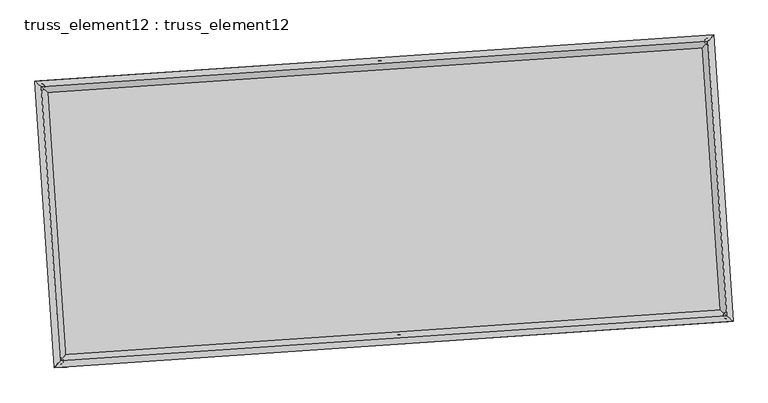
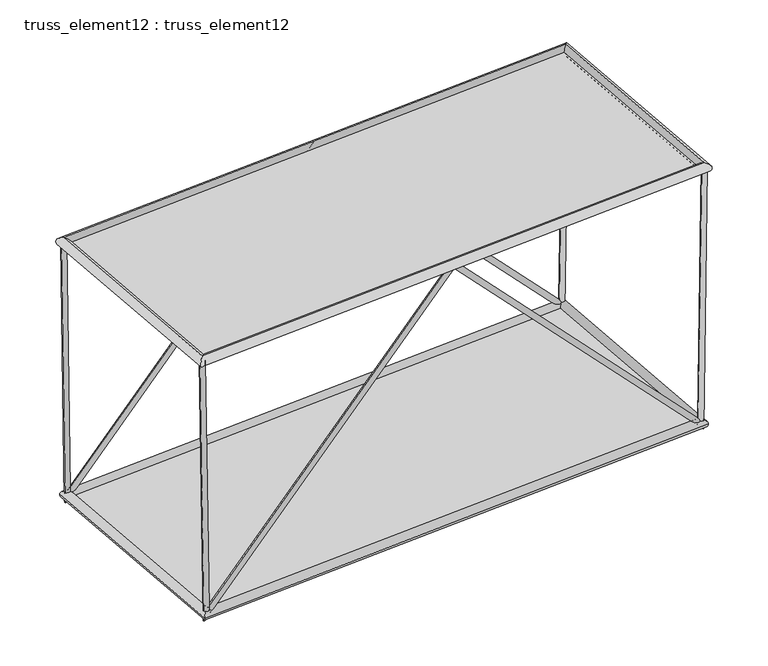
"""IFC4 building model written with IfcOpenShell, lengths in millimetres: plate geometry, truss_element12 : truss_element12."""

from ifc_helpers import new_model, si_unit, frame, origin, origin_with_axes, place, context, project, spatial, polyline, circle_curve, ellipse_curve, outline, extrude, source, transform, mapped, element, save
from ifc_brep_helpers import plane_surface, cylinder_surface, advanced_brep


def truss_element12_truss_element12_87516094(model_context):
    return source(origin(), model_context, "Body", "SolidModel", [
        advanced_brep(
        [(-3739.4843414, 2271.1412017, 5000.1872867), (-3838.5765897, 2257.7806857, 4998.6963313), (-3666.7596998, 2276.1000186, 122.3078972), (-3762.227183, 2262.9866615, -122.3078972), (1063.0583794, 2598.6083337, 5071.5713796), (1063.5164535, 2592.0357757, 4927.3317201), (5794.1667617, 2921.2046296, 122.3170383), (5890.5942153, 2921.1758589, -122.3170383), (5865.6107768, 2926.0761254, 5000.1936444), (5965.5998202, 2926.2902059, 4998.7289371)],
        [
            (0, 1, circle_curve(frame((-3789.0304655, 2264.4609437, 4999.441809), z_axis=(-0.01490740482663817, -0.0010164792667785262, 0.999888361794073), x_axis=(-0.13360539978853184, 0.9910341205011933, -0.0009844540481966856)), 50.0)),
            (1, 0, circle_curve(frame((-3789.0304655, 2264.4609437, 4999.441809), z_axis=(-0.01490740482663817, -0.0010164792667785262, 0.999888361794073), x_axis=(-0.13360539978853184, 0.9910341205011933, -0.0009844540481966856)), 50.0)),
            (0, 2),
            (2, 3, ellipse_curve(frame((-3714.4934414, 2269.54334, 0.0), z_axis=(-0.9285444803963763, -0.06331391839020976, 0.3657820329971138), x_axis=(0.3649346609037332, 0.024883507280505895, 0.93070054493188)), 131.701033, 50.0)),
            (3, 1),
            (3, 2, ellipse_curve(frame((-3714.4934414, 2269.54334, 0.0), z_axis=(-0.9285444803963763, -0.06331391839020976, 0.3657820329971138), x_axis=(0.3649346609037332, 0.024883507280505895, 0.93070054493188)), 131.701033, 50.0)),
            (2, 4),
            (4, 5, ellipse_curve(frame((1063.2874165, 2595.3220547, 4999.4515499), z_axis=(-0.9976833937280465, -0.06802823806868136, -6.858978492521302e-05), x_axis=(6.843088956005366e-05, 4.666042230024793e-06, -0.9999999976477206)), 72.2768712, 50.0)),
            (5, 3),
            (5, 4, ellipse_curve(frame((1063.2874165, 2595.3220547, 4999.4515499), z_axis=(-0.9976833937280465, -0.06802823806868136, -6.858978492521302e-05), x_axis=(6.843088956005366e-05, 4.666042230024793e-06, -0.9999999976477206)), 72.2768712, 50.0)),
            (4, 6),
            (6, 7, ellipse_curve(frame((5842.3804885, 2921.1902443, 0.0), z_axis=(-0.9284714273096886, -0.06330893717792861, -0.36596828707267914), x_axis=(-0.3651204835023758, -0.02489617781713149, 0.9306273222171639)), 131.7212392, 50.0)),
            (7, 5),
            (7, 6, ellipse_curve(frame((5842.3804885, 2921.1902443, 0.0), z_axis=(-0.9284714273096886, -0.06330893717792861, -0.36596828707267914), x_axis=(-0.3651204835023758, -0.02489617781713149, 0.9306273222171639)), 131.7212392, 50.0)),
            (8, 9, circle_curve(frame((5915.6052985, 2926.1831657, 4999.4612908), z_axis=(0.0146449619914404, 0.0009985842874829112, 0.9998922581546925), x_axis=(-0.0021552007044751543, 0.9999972098877479, -0.0009671228685221853)), 50.0)),
            (9, 8, circle_curve(frame((5915.6052985, 2926.1831657, 4999.4612908), z_axis=(0.0146449619914404, 0.0009985842874829112, 0.9998922581546925), x_axis=(-0.0021552007044751543, 0.9999972098877479, -0.0009671228685221853)), 50.0)),
            (6, 8),
            (9, 7),
        ],
        [
            plane_surface(frame((-3789.0304655, 2314.4609179, 4999.4926386), z_axis=(-0.014907404826640259, -0.0010164792667773047, 0.9998883617940729), x_axis=(0.9998888784666697, -1.5154751946688795e-05, 0.014907397123536715))),
            cylinder_surface(frame((-3789.0304655, 2264.4609437, 4999.441809), z_axis=(-0.01490740482663817, -0.0010164792667785262, 0.999888361794073), x_axis=(-0.13360539978853184, 0.9910341205011933, -0.0009844540481966856)), 50.0),
            cylinder_surface(frame((-3714.4934414, 2269.54334, 0.0), z_axis=(-0.6901322286195807, -0.04705749323136387, -0.7221517149126984), x_axis=(-0.020411728114871647, 0.9987523666831909, -0.04557489879406897)), 50.0),
            cylinder_surface(frame((1063.2874165, 2595.3220547, 4999.4515499), z_axis=(-0.6902310570943108, -0.04706423196937507, 0.722056816248973), x_axis=(-0.11534289058656251, 0.9922793715813788, -0.04558142522124768)), 50.0),
            plane_surface(frame((5915.6052985, 2876.1831906, 4999.5112253), z_axis=(0.014644961991439494, 0.000998584287486898, 0.9998922581546924), x_axis=(0.999892756793582, -1.462579745314941e-05, -0.014644954688108676))),
            cylinder_surface(frame((5842.3804885, 2921.1902443, 0.0), z_axis=(-0.0146449619914404, -0.0009985842874829112, -0.9998922581546925), x_axis=(-0.0021552007044751543, 0.9999972098877479, -0.0009671228685221853)), 50.0),
        ],
        [
            (0, [[1, 2]]),
            (1, [[-1, 3, 4, 5]]),
            (1, [[-2, -5, 6, -3]]),
            (2, [[-4, 7, 8, 9]]),
            (2, [[-6, -9, 10, -7]]),
            (3, [[-8, 11, 12, 13]]),
            (3, [[-10, -13, 14, -11]]),
            (4, [[15, 16]]),
            (5, [[-12, 17, -16, 18]]),
            (5, [[-14, -18, -15, -17]]),
        ],
    ),
        advanced_brep(
        [(-3467.3713885, -1719.5923826, 5000.1872867), (-3566.4636368, -1732.9528986, 4998.6963313), (-3394.6467469, -1714.6335657, 122.3078972), (-3490.1142301, -1727.7469228, -122.3078972), (1335.1713323, -1392.1252506, 5071.5713796), (1335.6294064, -1398.6978086, 4927.3317201), (6066.2797147, -1069.5289547, 122.3170383), (6162.7071682, -1069.5577254, -122.3170383), (6137.7237297, -1064.6574589, 5000.1936444), (6237.7127731, -1064.4433784, 4998.7289371)],
        [
            (0, 1, circle_curve(frame((-3516.9175126, -1726.2726406, 4999.441809), z_axis=(-0.014907404826637962, -0.0010164792667784767, 0.999888361794073), x_axis=(-0.13360539978853184, 0.9910341205011933, -0.0009844540481967064)), 50.0)),
            (1, 0, circle_curve(frame((-3516.9175126, -1726.2726406, 4999.441809), z_axis=(-0.014907404826637962, -0.0010164792667784767, 0.999888361794073), x_axis=(-0.13360539978853184, 0.9910341205011933, -0.0009844540481967064)), 50.0)),
            (0, 2),
            (2, 3, ellipse_curve(frame((-3442.3804885, -1721.1902443, 0.0), z_axis=(-0.9285444803963764, -0.0633139183902097, 0.36578203299711326), x_axis=(0.36493466090373267, 0.024883507280505864, 0.9307005449318803)), 131.701033, 50.0)),
            (3, 1),
            (3, 2, ellipse_curve(frame((-3442.3804885, -1721.1902443, 0.0), z_axis=(-0.9285444803963764, -0.0633139183902097, 0.36578203299711326), x_axis=(0.36493466090373267, 0.024883507280505864, 0.9307005449318803)), 131.701033, 50.0)),
            (2, 4),
            (4, 5, ellipse_curve(frame((1335.4003694, -1395.4115296, 4999.4515499), z_axis=(-0.9976833937280466, -0.06802823806868125, -6.858978492569457e-05), x_axis=(6.843088956082234e-05, 4.6660422299959605e-06, -0.9999999976477206)), 72.2768712, 50.0)),
            (5, 3),
            (5, 4, ellipse_curve(frame((1335.4003694, -1395.4115296, 4999.4515499), z_axis=(-0.9976833937280466, -0.06802823806868125, -6.858978492569457e-05), x_axis=(6.843088956082234e-05, 4.6660422299959605e-06, -0.9999999976477206)), 72.2768712, 50.0)),
            (4, 6),
            (6, 7, ellipse_curve(frame((6114.4934414, -1069.54334, 0.0), z_axis=(-0.9284714273096886, -0.06330893717792847, -0.36596828707267864), x_axis=(-0.3651204835023754, -0.024896177817131368, 0.930627322217164)), 131.7212392, 50.0)),
            (7, 5),
            (7, 6, ellipse_curve(frame((6114.4934414, -1069.54334, 0.0), z_axis=(-0.9284714273096886, -0.06330893717792847, -0.36596828707267864), x_axis=(-0.3651204835023754, -0.024896177817131368, 0.930627322217164)), 131.7212392, 50.0)),
            (8, 9, circle_curve(frame((6187.7182514, -1064.5504186, 4999.4612908), z_axis=(0.014644961991440565, 0.0009985842874829474, 0.9998922581546924), x_axis=(-0.0021552007044752385, 0.999997209887748, -0.0009671228685222203)), 50.0)),
            (9, 8, circle_curve(frame((6187.7182514, -1064.5504186, 4999.4612908), z_axis=(0.014644961991440565, 0.0009985842874829474, 0.9998922581546924), x_axis=(-0.0021552007044752385, 0.999997209887748, -0.0009671228685222203)), 50.0)),
            (6, 8),
            (9, 7),
        ],
        [
            plane_surface(frame((-3516.9175126, -1676.2726664, 4999.4926386), z_axis=(-0.014907404826640259, -0.001016479266777302, 0.9998883617940729), x_axis=(0.9998888784666697, -1.5154751946688795e-05, 0.014907397123536715))),
            cylinder_surface(frame((-3516.9175126, -1726.2726406, 4999.441809), z_axis=(-0.014907404826637962, -0.0010164792667784767, 0.999888361794073), x_axis=(-0.13360539978853184, 0.9910341205011933, -0.0009844540481967064)), 50.0),
            cylinder_surface(frame((-3442.3804885, -1721.1902443, 0.0), z_axis=(-0.6901322286195796, -0.04705749323136377, -0.7221517149126994), x_axis=(-0.020411728114871578, 0.9987523666831909, -0.04557489879406886)), 50.0),
            cylinder_surface(frame((1335.4003694, -1395.4115296, 4999.4515499), z_axis=(-0.6902310570943105, -0.047064231969374926, 0.7220568162489734), x_axis=(-0.11534289058656241, 0.9922793715813789, -0.04558142522124771)), 50.0),
            plane_surface(frame((6187.7182514, -1114.5503937, 4999.5112253), z_axis=(0.014644961991439493, 0.0009985842874868942, 0.9998922581546924), x_axis=(0.999892756793582, -1.462579745270532e-05, -0.014644954688108676))),
            cylinder_surface(frame((6114.4934414, -1069.54334, 0.0), z_axis=(-0.014644961991440568, -0.0009985842874829477, -0.9998922581546926), x_axis=(-0.0021552007044752385, 0.999997209887748, -0.0009671228685222203)), 50.0),
        ],
        [
            (0, [[1, 2]]),
            (1, [[-1, 3, 4, 5]]),
            (1, [[-2, -5, 6, -3]]),
            (2, [[-4, 7, 8, 9]]),
            (2, [[-6, -9, 10, -7]]),
            (3, [[-8, 11, 12, 13]]),
            (3, [[-10, -13, 14, -11]]),
            (4, [[15, 16]]),
            (5, [[-12, 17, -16, 18]]),
            (5, [[-14, -18, -15, -17]]),
        ],
    ),
        advanced_brep(
        [(-3516.9124119, -1726.2669872, 4909.4418091), (-3516.9226134, -1726.2782939, 5089.4418088), (-3789.0362865, 2264.4658524, 5089.4418088), (-3789.0246446, 2264.4560351, 4909.4418091), (5915.6100395, 2926.1887945, 5089.4612906), (5915.6005574, 2926.1775369, 4909.4612909), (6187.7237126, -1064.5553518, 5089.4612906), (6187.7127901, -1064.5454854, 4909.4612909)],
        [
            (0, 1, ellipse_curve(frame((-3516.9175126, -1726.2726406, 4999.441809), z_axis=(-0.7535719234040453, 0.6573654662781746, -1.4162099958110805e-06), x_axis=(-0.6573654662766633, -0.7535719234053638, -1.4162100019367133e-06)), 127.2792206, 90.0)),
            (1, 2),
            (2, 3, ellipse_curve(frame((-3789.0304655, 2264.4609437, 4999.441809), z_axis=(-0.6573654662766631, -0.7535719234053638, -1.4162100006772274e-06), x_axis=(0.7535719234040454, -0.6573654662781746, 1.4162099945515952e-06)), 127.2792206, 90.0)),
            (3, 0),
            (1, 0, ellipse_curve(frame((-3516.9175126, -1726.2726406, 4999.441809), z_axis=(-0.7535719234040453, 0.6573654662781746, -1.4162099958110805e-06), x_axis=(-0.6573654662766633, -0.7535719234053638, -1.4162100019367133e-06)), 127.2792206, 90.0)),
            (3, 2, ellipse_curve(frame((-3789.0304655, 2264.4609437, 4999.441809), z_axis=(-0.6573654662766631, -0.7535719234053638, -1.4162100006772274e-06), x_axis=(0.7535719234040454, -0.6573654662781746, 1.4162099945515952e-06)), 127.2792206, 90.0)),
            (2, 4),
            (4, 5, ellipse_curve(frame((5915.6052985, 2926.1831657, 4999.4612908), z_axis=(-0.7535719234040438, 0.6573654662781764, -1.4162099976144125e-06), x_axis=(-0.657365466276665, -0.753571923405362, -1.4162099976144098e-06)), 127.2792206, 90.0)),
            (5, 3),
            (5, 4, ellipse_curve(frame((5915.6052985, 2926.1831657, 4999.4612908), z_axis=(-0.7535719234040438, 0.6573654662781764, -1.4162099976144125e-06), x_axis=(-0.657365466276665, -0.753571923405362, -1.4162099976144098e-06)), 127.2792206, 90.0)),
            (4, 6),
            (6, 7, ellipse_curve(frame((6187.7182514, -1064.5504186, 4999.4612908), z_axis=(0.657365466276665, 0.753571923405362, 1.4162099988738953e-06), x_axis=(-0.7535719234040437, 0.6573654662781766, -1.4162099988738978e-06)), 127.2792206, 90.0)),
            (7, 5),
            (7, 6, ellipse_curve(frame((6187.7182514, -1064.5504186, 4999.4612908), z_axis=(0.657365466276665, 0.753571923405362, 1.4162099988738953e-06), x_axis=(-0.7535719234040437, 0.6573654662781766, -1.4162099988738978e-06)), 127.2792206, 90.0)),
            (6, 1),
            (0, 7),
        ],
        [
            cylinder_surface(frame((-3516.9175126, -1726.2726406, 4999.441809), z_axis=(0.06802823822870717, -0.9976833960748764, 0.0), x_axis=(-0.9976833942298226, -0.06802823810289996, -6.081673841992654e-05)), 90.0),
            cylinder_surface(frame((-3789.0304655, 2264.4609437, 4999.441809), z_axis=(-0.9976833960728758, -0.06802823822856607, -2.0028233857946695e-06), x_axis=(-0.06802823799352406, 0.9976833943573583, -5.881391503326435e-05)), 90.0),
            cylinder_surface(frame((5915.6052985, 2926.1831657, 4999.4612908), z_axis=(-0.06802823822870217, 0.9976833960748768, 0.0), x_axis=(0.997683394464865, 0.06802823811892159, -5.6811091650933643e-05)), 90.0),
            cylinder_surface(frame((6187.7182514, -1064.5504186, 4999.4612908), z_axis=(0.9976833960728758, 0.06802823822856596, 2.002823387575851e-06), x_axis=(0.06802823822856595, -0.9976833943413317, -5.881391503504554e-05)), 90.0),
        ],
        [
            (0, [[1, 2, 3, 4]]),
            (0, [[5, -4, 6, -2]]),
            (1, [[-3, 7, 8, 9]]),
            (1, [[-6, -9, 10, -7]]),
            (2, [[-8, 11, 12, 13]]),
            (2, [[-10, -13, 14, -11]]),
            (3, [[-12, 15, -1, 16]]),
            (3, [[-14, -16, -5, -15]]),
        ],
    ),
        advanced_brep(
        [(-3358.7115243, -1625.2761972, 0.0), (-3526.0494527, -1817.1042913, 0.0), (-3810.4074885, 2353.2123043, 0.0), (-3618.5793943, 2185.8743758, 0.0), (5926.0494527, 3017.1042913, 0.0), (5758.7115243, 2825.2761972, 0.0), (6210.4074885, -1153.2123043, 0.0), (6018.5793943, -985.8743758, 0.0)],
        [
            (0, 1, ellipse_curve(frame((-3442.3804885, -1721.1902443, 0.0), z_axis=(-0.7535719234054605, 0.6573654662780778, 0.0), x_axis=(-0.6573654662780778, -0.7535719234054605, 0.0)), 127.2792206, 90.0)),
            (1, 2),
            (2, 3, ellipse_curve(frame((-3714.4934414, 2269.54334, 0.0), z_axis=(-0.6573654662780778, -0.7535719234054605, 0.0), x_axis=(0.7535719234054605, -0.6573654662780779, 0.0)), 127.2792206, 90.0)),
            (3, 0),
            (1, 0, ellipse_curve(frame((-3442.3804885, -1721.1902443, 0.0), z_axis=(-0.7535719234054605, 0.6573654662780778, 0.0), x_axis=(-0.6573654662780778, -0.7535719234054605, 0.0)), 127.2792206, 90.0)),
            (3, 2, ellipse_curve(frame((-3714.4934414, 2269.54334, 0.0), z_axis=(-0.6573654662780778, -0.7535719234054605, 0.0), x_axis=(0.7535719234054605, -0.6573654662780779, 0.0)), 127.2792206, 90.0)),
            (2, 4),
            (4, 5, ellipse_curve(frame((5842.3804885, 2921.1902443, 0.0), z_axis=(-0.7535719234054591, 0.6573654662780795, 0.0), x_axis=(-0.6573654662780795, -0.7535719234054591, 0.0)), 127.2792206, 90.0)),
            (5, 3),
            (5, 4, ellipse_curve(frame((5842.3804885, 2921.1902443, 0.0), z_axis=(-0.7535719234054591, 0.6573654662780795, 0.0), x_axis=(-0.6573654662780795, -0.7535719234054591, 0.0)), 127.2792206, 90.0)),
            (4, 6),
            (6, 7, ellipse_curve(frame((6114.4934414, -1069.54334, 0.0), z_axis=(0.6573654662780795, 0.7535719234054591, 0.0), x_axis=(-0.7535719234054591, 0.6573654662780795, 0.0)), 127.2792206, 90.0)),
            (7, 5),
            (7, 6, ellipse_curve(frame((6114.4934414, -1069.54334, 0.0), z_axis=(0.6573654662780795, 0.7535719234054591, 0.0), x_axis=(-0.7535719234054591, 0.6573654662780795, 0.0)), 127.2792206, 90.0)),
            (6, 1),
            (0, 7),
        ],
        [
            cylinder_surface(frame((-3442.3804885, -1721.1902443, 0.0), z_axis=(0.06802823822870757, -0.9976833960748761, 0.0), x_axis=(-0.9976833960748761, -0.06802823822870757, 0.0)), 90.0),
            cylinder_surface(frame((-3714.4934414, 2269.54334, 0.0), z_axis=(-0.9976833960748764, -0.06802823822870287, 0.0), x_axis=(-0.06802823822870287, 0.9976833960748764, 0.0)), 90.0),
            cylinder_surface(frame((5842.3804885, 2921.1902443, 0.0), z_axis=(-0.06802823822870313, 0.9976833960748764, 0.0), x_axis=(0.9976833960748764, 0.06802823822870313, 0.0)), 90.0),
            cylinder_surface(frame((6114.4934414, -1069.54334, 0.0), z_axis=(0.9976833960748764, 0.06802823822870296, 0.0), x_axis=(0.06802823822870296, -0.9976833960748764, 0.0)), 90.0),
        ],
        [
            (0, [[1, 2, 3, 4]]),
            (0, [[5, -4, 6, -2]]),
            (1, [[-3, 7, 8, 9]]),
            (1, [[-6, -9, 10, -7]]),
            (2, [[-8, 11, 12, 13]]),
            (2, [[-10, -13, 14, -11]]),
            (3, [[-12, 15, -1, 16]]),
            (3, [[-14, -16, -5, -15]]),
        ],
    ),
        extrude(outline(polyline([(-3442.3804885, -1721.1902443), (-3714.4934414, 2269.54334), (5842.3804885, 2921.1902443), (6114.4934414, -1069.54334), (-3442.3804885, -1721.1902443)])), origin_with_axes(), (0.0, 0.0, 1.0), 20.0),
        extrude(outline(polyline([(-2000.0000001, 4863.5848818), (1999.9999999, 4863.5848818), (2000.0, -4863.5848819), (-2000.0, -4863.5848819), (-2000.0000001, 4863.5848818)])), frame((1199.3438929, 599.9552626, 4999.4515499), z_axis=(-1.9981836369831424e-06, -1.3624855074029978e-07, 0.9999999999979944), x_axis=(-0.06802823822870725, 0.9976833960748762, 0.0)), (0.0, 0.0, 1.0), 20.0),
    ])


if __name__ == "__main__":
    model = new_model("IFC4")
    model_context = context("Model", 3, world=origin())
    ifc_project = project(units=[si_unit("LENGTHUNIT", "METRE", prefix="MILLI")], contexts=[model_context])
    site = spatial("IfcSite", under=ifc_project)
    building = spatial("IfcBuilding", under=site)
    placement = place(None, origin())
    truss_element12_truss_element12_shape = truss_element12_truss_element12_87516094(model_context)
    element("IfcPlate", 1, ObjectType="truss_element12 : truss_element12", at=placement, inside=building, context=model_context, shape_type="MappedRepresentation", body=[
        mapped(truss_element12_truss_element12_shape, transform((0.0, 0.0, 0.0), x_axis=(1.0, 0.0, 0.0), y_axis=(0.0, 1.0, 0.0), z_axis=(0.0, 0.0, 1.0))),
    ])
    save(model, "model.ifc")

# Revit data of these elements
# Type "truss_element12 : truss_element12"
#   steellbar1 = 90 mm
#   steelbar2 = 50 mm
#   offset1 = 5000 mm
#   M = Default Roof
# Element 1 (IfcPlate, "truss_element12 : truss_element12")
#   Materials on its faces: "Default Roof"
# Materials
#   "Default Roof": class "Miscellaneous", colour RGB 0 127 0, transparency 0, Comments = "Rendering appearance not upgraded Rendering appearance not upgraded ", Cost = 0
